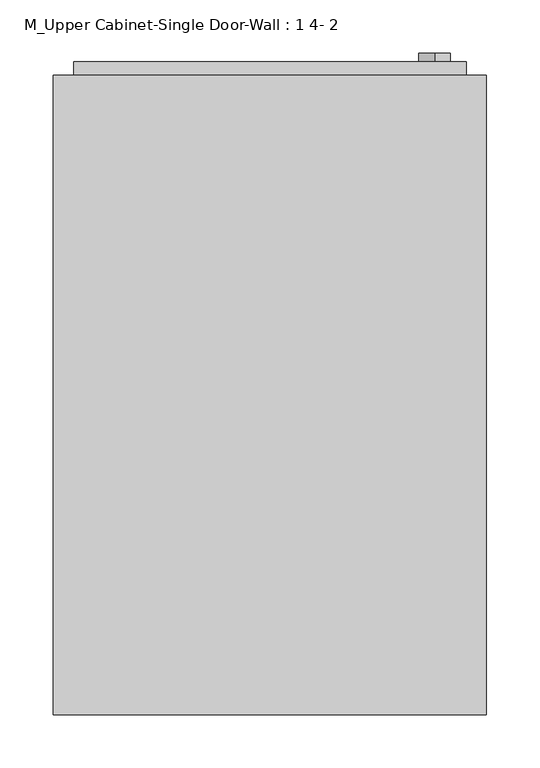
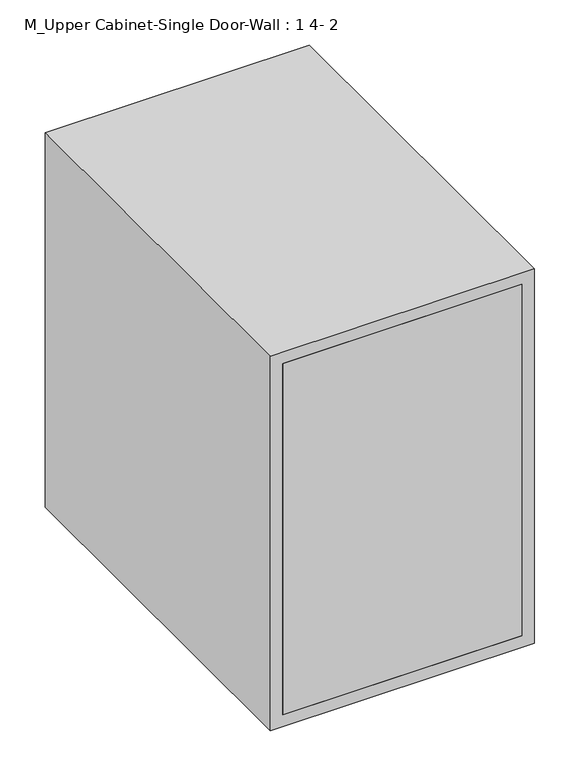
"""IFC4 building model written with IfcOpenShell, lengths in millimetres: furniture geometry, M_Upper Cabinet-Single Door-Wall : 1 4- 2."""

from ifc_helpers import new_model, si_unit, point, frame, frame_2d, origin, place, context, project, spatial, polyline, circle_curve, trimmed, segment, composite_curve, outline, extrude, source, transform, mapped, element, save


def m_upper_cabinet_single_door_wall_1_4_2_264910c1(model_context):
    return source(origin(), model_context, "Body", "SweptSolid", [
        extrude(outline(polyline([(-154.3788372, 669.8257813), (213.9211628, 669.8257813), (213.9211628, 638.0757813), (-154.3788372, 638.0757813), (-154.3788372, 669.8257813)])), frame((0.0, 0.0, 1409.45), z_axis=(0.0, 0.0, 1.0), x_axis=(1.0, 0.0, 0.0)), (0.0, 0.0, 1.0), 571.5),
        extrude(outline(polyline([(213.9211628, 57.15), (-154.3788372, 57.15), (-154.3788372, 76.2), (213.9211628, 76.2), (213.9211628, 57.15)])), frame((0.0, 0.0, 1409.45), z_axis=(0.0, 0.0, 1.0), x_axis=(1.0, 0.0, 0.0)), (0.0, 0.0, 1.0), 571.5),
        extrude(outline(polyline([(2000.0, -173.4288372), (1390.4, -173.4288372), (1390.4, 232.9711628), (2000.0, 232.9711628), (2000.0, -173.4288372)]), holes=[polyline([(1980.95, -154.3788372), (1980.95, 213.9211628), (1409.45, 213.9211628), (1409.45, -154.3788372), (1980.95, -154.3788372)])]), frame((0.0, 57.15, 0.0), z_axis=(0.0, 1.0, 0.0), x_axis=(0.0, 0.0, 1.0)), (0.0, 0.0, 1.0), 599.9757812),
        extrude(outline(composite_curve([segment(trimmed(circle_curve(frame_2d((1585.4953371, 184.3613252)), 15.0), [point((1570.4953371, 184.3613252))], [point((1600.4953371, 184.3613252))], False, "CARTESIAN"), True, "CONTINUOUS"), segment(trimmed(circle_curve(frame_2d((1585.4953371, 184.3613252)), 15.0), [point((1600.4953371, 184.3613252))], [point((1570.4953371, 184.3613252))], False, "CARTESIAN"), True, "CONTINUOUS")], self_intersect=False)), frame((0.0, 669.8257813, 0.0), z_axis=(0.0, 1.0, 0.0), x_axis=(0.0, 0.0, 1.0)), (0.0, 0.0, 1.0), 8.0),
    ])


if __name__ == "__main__":
    model = new_model("IFC4")
    model_context = context("Model", 3, world=origin())
    ifc_project = project(units=[si_unit("LENGTHUNIT", "METRE", prefix="MILLI")], contexts=[model_context])
    site = spatial("IfcSite", under=ifc_project)
    building = spatial("IfcBuilding", under=site)
    placement = place(None, origin())
    m_upper_cabinet_single_door_wall_1_4_2_shape = m_upper_cabinet_single_door_wall_1_4_2_264910c1(model_context)
    element("IfcFurniture", 1, ObjectType="M_Upper Cabinet-Single Door-Wall : 1 4- 2", at=placement, inside=building, context=model_context, shape_type="MappedRepresentation", body=[
        mapped(m_upper_cabinet_single_door_wall_1_4_2_shape, transform((0.0, 0.0, 0.0), x_axis=(1.0, 0.0, 0.0), y_axis=(0.0, 1.0, 0.0), z_axis=(0.0, 0.0, 1.0))),
    ])
    save(model, "model.ifc")

# Revit data of these elements
# Type "M_Upper Cabinet-Single Door-Wall : 1 4- 2"
#   Depth = 1' - 11 159/256"
#   Height = 2' - 0"
#   Top Of Cabinet = 6' - 6.74016"
#   Width = 1' - 4"
#   Cabinet Material = Base cabinet 2120100 Aspekt - 83012120100 - White
#   Door/Drawer Material = Base cabinet 2120100 Aspekt - 83012120100 - White
#   Handle Material = Cabinets - Handles
#   Default Elevation = 0
# Element 1 (IfcFurniture, "M_Upper Cabinet-Single Door-Wall : 1 4- 2")
#   Materials on its faces: "Base cabinet 2120100 Aspekt - 83012120100 - White"
# Materials
#   "Base cabinet 2120100 Aspekt - 83012120100 - White": class "Miscellaneous", colour RGB 255 255 255, transparency 0, Manufacturer = "Marbodal", URL = "http://www.marbodal.se", Cost = 0
#   "Cabinets - Handles": class "Metal", colour RGB 57 57 57, transparency 0
